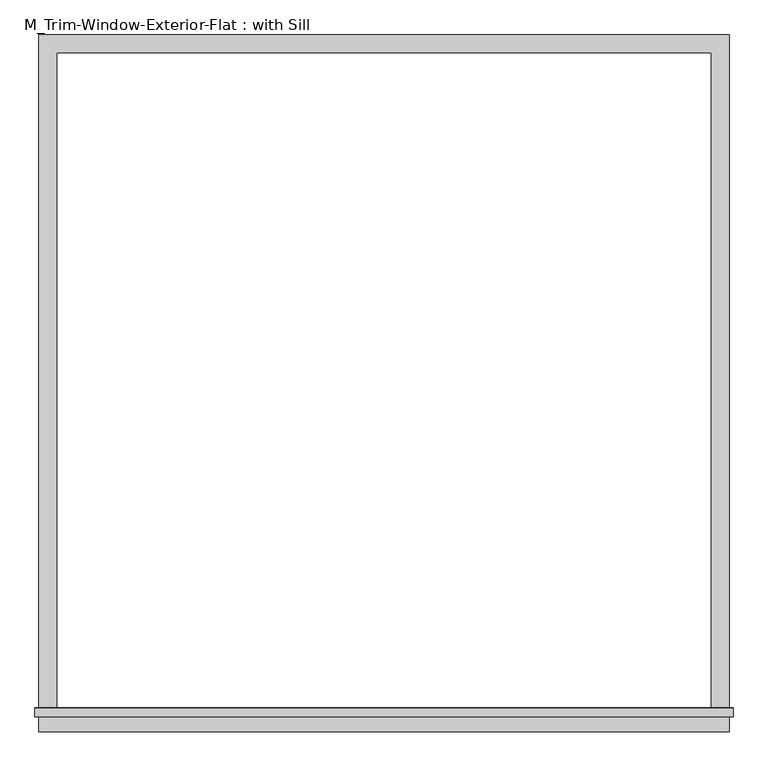
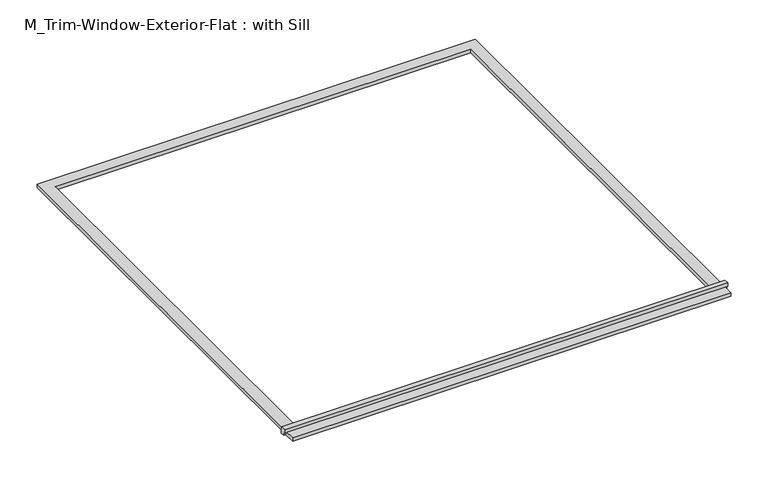
"""IFC4 building model written with IfcOpenShell, lengths in millimetres: proxy geometry, M_Trim-Window-Exterior-Flat : with Sill."""

from ifc_helpers import new_model, si_unit, frame, origin, origin_with_axes, place, context, project, spatial, polyline, outline, extrude, source, transform, mapped, element, save


def m_trim_window_exterior_flat_with_sill_58d19bd2(model_context):
    return source(origin(), model_context, "Body", "SweptSolid", [
        extrude(outline(polyline([(1160.0, -2220.4323709), (1160.0, -2280.4323709), (-1160.0, -2280.4323709), (-1160.0, -2220.4323709), (1160.0, -2220.4323709)])), origin_with_axes(), (0.0, 0.0, 1.0), 19.05),
        extrude(outline(polyline([(-2230.0, 38.1), (-2202.4580645, 38.1), (-2200.0, 19.05), (-2200.0, 0.0), (-2220.4323709, 0.0), (-2220.4323709, 19.05), (-2230.0, 19.05), (-2230.0, 38.1)])), frame((-1172.7, 0.0, 0.0), z_axis=(1.0, 0.0, 0.0), x_axis=(0.0, 1.0, 0.0)), (0.0, 0.0, 1.0), 2345.4),
        extrude(outline(polyline([(-1160.0, 60.0), (1160.0, 60.0), (1160.0, -2200.0), (1100.0, -2200.0), (1100.0, 0.0), (-1100.0, 0.0), (-1100.0, -2200.0), (-1160.0, -2200.0), (-1160.0, 60.0)])), origin_with_axes(), (0.0, 0.0, 1.0), 19.05),
    ])


if __name__ == "__main__":
    model = new_model("IFC4")
    model_context = context("Model", 3, world=origin())
    ifc_project = project(units=[si_unit("LENGTHUNIT", "METRE", prefix="MILLI")], contexts=[model_context])
    site = spatial("IfcSite", under=ifc_project)
    building = spatial("IfcBuilding", under=site)
    placement = place(None, origin())
    m_trim_window_exterior_flat_with_sill_shape = m_trim_window_exterior_flat_with_sill_58d19bd2(model_context)
    element("IfcBuildingElementProxy", 1, Name="M_Trim-Window-Exterior-Flat : with Sill", ObjectType="M_Trim-Window-Exterior-Flat : with Sill", at=placement, inside=building, context=model_context, shape_type="MappedRepresentation", body=[
        mapped(m_trim_window_exterior_flat_with_sill_shape, transform((0.0, 0.0, 0.0), x_axis=(1.0, 0.0, 0.0), y_axis=(0.0, 1.0, 0.0), z_axis=(0.0, 0.0, 1.0))),
    ])
    save(model, "model.ifc")

# Revit data of these elements
# Type "M_Trim-Window-Exterior-Flat : with Sill"
#   Trim Width = 0.06 m
#   Trim Thickness_Picture Frame = 0.03 m
#   Trim Thickness_with Sill = 0.01905 m
#   Sill Thickness = 0.03 m
#   Opening Width [instance default] = 0.60 m
#   Opening Height [instance default] = 0.90 m
#   Default Elevation = 1.20 m
#   Sill = yes
#   Picture Frame = no
#   Trim Material [instance default] = none
# Element 1 (IfcBuildingElementProxy, "M_Trim-Window-Exterior-Flat : with Sill")
#   Opening Width = 2.20 m
#   Opening Height = 2.20 m
#   Trim Material = Clad - White
#   Materials on its faces: "Clad - White"
# Materials
#   "Clad - White": class "Wood", colour RGB 242 242 238, transparency 0, Cost = 0
